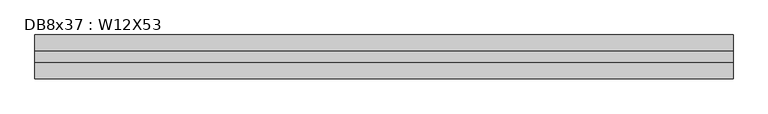
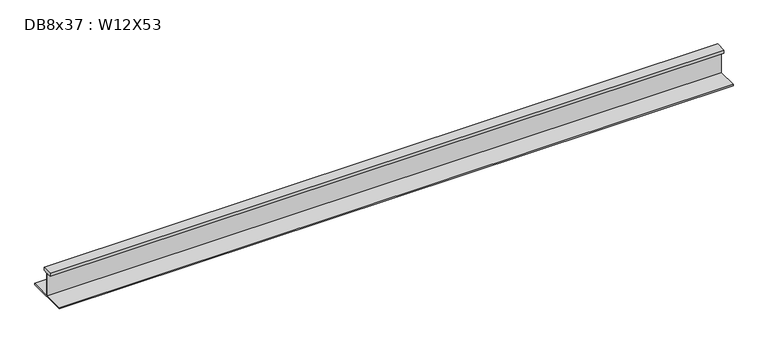
"""IFC4 building model written with IfcOpenShell, lengths in millimetres: beam geometry, DB8x37 : W12X53."""

import ifcopenshell
import ifcopenshell.guid

model = None  # the IFC model being written
_history = None  # IfcOwnerHistory: only IFC2X3 demands one
_inside = {}  # id of a spatial element -> (the spatial element, [elements in it])
_under = {}  # id of a project, library or spatial element -> (it, [spatial elements below it])
_declared = {}  # id of a project -> (the project, [libraries it declares])
_typed = {}  # id of a type object -> (the type object, [elements of that type])
_made_of = {}  # id of a material, layer set ... -> (it, [elements and type objects made of it])


def new_model(schema):
    """Start an empty IFC model of exactly this schema.

    Asked for "IFC4X3", IfcOpenShell would pick the latest addendum, in which some entities
    have other attributes; the version numbers below select the first issue.
    IFC2X3 requires an IfcOwnerHistory on every rooted entity: one is made here for all.
    """
    global model, _history
    if schema == "IFC4X3":
        model = ifcopenshell.file(schema_version=(4, 3, 0, 0))
    else:
        model = ifcopenshell.file(schema=schema)
    _inside.clear()
    _under.clear()
    _declared.clear()
    _typed.clear()
    _made_of.clear()
    _history = None
    if model.schema == "IFC2X3":
        org = make("IfcOrganization", Name="unknown")
        user = make(
            "IfcPersonAndOrganization",
            ThePerson=make("IfcPerson", FamilyName="unknown"),
            TheOrganization=org,
        )
        app = make(
            "IfcApplication",
            ApplicationDeveloper=org,
            Version="unknown",
            ApplicationFullName="unknown",
            ApplicationIdentifier="unknown",
        )
        _history = make(
            "IfcOwnerHistory",
            OwningUser=user,
            OwningApplication=app,
            ChangeAction="ADDED",
            CreationDate=0,
        )
    return model


def make(cls, **values):
    """One entity of the class cls with the attributes given. An attribute that is None is left unset."""
    return model.create_entity(
        cls, **{name: value for name, value in values.items() if value is not None}
    )


def rooted(cls, **values):
    """An entity with a GlobalId (a new one), such as an element, a storey or a relation."""
    return make(cls, GlobalId=ifcopenshell.guid.new(), OwnerHistory=_history, **values)


def si_unit(unit_type, name, prefix=None):
    """IfcSIUnit, for example si_unit("LENGTHUNIT", "METRE", prefix="MILLI")."""
    return make("IfcSIUnit", UnitType=unit_type, Prefix=prefix, Name=name)


def assignment(units):
    """IfcUnitAssignment: the units of a project."""
    return None if units is None else make("IfcUnitAssignment", Units=units)


def point(xyz):
    """IfcCartesianPoint."""
    return None if xyz is None else make("IfcCartesianPoint", Coordinates=xyz)


def direction(xyz):
    """IfcDirection."""
    return None if xyz is None else make("IfcDirection", DirectionRatios=xyz)


def frame(location, z_axis=None, x_axis=None):
    """IfcAxis2Placement3D, a coordinate frame: its origin and axes. An axis left out is left unset."""
    return make(
        "IfcAxis2Placement3D",
        Location=point(location),
        Axis=direction(z_axis),
        RefDirection=direction(x_axis),
    )


def origin():
    """The frame at (0, 0, 0) with its axes left unset."""
    return frame((0.0, 0.0, 0.0))


def place(relative_to, where):
    """IfcLocalPlacement: puts the frame where relative to a parent placement (None: the world)."""
    return make(
        "IfcLocalPlacement", PlacementRelTo=relative_to, RelativePlacement=where
    )


def context(
    kind, dimensions, precision=None, world=None, true_north=None, identifier=None
):
    """IfcGeometricRepresentationContext, for example the 3D "Model" context."""
    return make(
        "IfcGeometricRepresentationContext",
        ContextIdentifier=identifier,
        ContextType=kind,
        CoordinateSpaceDimension=dimensions,
        Precision=precision,
        WorldCoordinateSystem=world,
        TrueNorth=true_north,
    )


def project(units=None, contexts=None):
    """IfcProject with its units and contexts."""
    return rooted(
        "IfcProject",
        Name="project",
        RepresentationContexts=contexts,
        UnitsInContext=assignment(units),
    )


def spatial(cls, under=None, at=None, **own):
    """A site, building, storey or space (cls), placed at a placement, below another one or the project."""
    s = rooted(cls, ObjectPlacement=at, **own)
    if under is not None:
        _under.setdefault(under.id(), (under, []))[1].append(s)
    return s


def polyline(points):
    """IfcPolyline through the points."""
    return make("IfcPolyline", Points=[point(p) for p in points])


def outline(outer, holes=None, kind="AREA"):
    """IfcArbitraryClosedProfileDef: a profile drawn as a closed curve; with holes, ...WithVoids."""
    if holes is None:
        return make("IfcArbitraryClosedProfileDef", ProfileType=kind, OuterCurve=outer)
    return make(
        "IfcArbitraryProfileDefWithVoids",
        ProfileType=kind,
        OuterCurve=outer,
        InnerCurves=holes,
    )


def extrude(swept, where, along, depth):
    """IfcExtrudedAreaSolid: the profile swept, set in the frame where, extruded along a direction by depth."""
    return make(
        "IfcExtrudedAreaSolid",
        SweptArea=swept,
        Position=where,
        ExtrudedDirection=direction(along),
        Depth=depth,
    )


def shape(context_of_items, identifier, shape_type, items):
    """IfcShapeRepresentation: the items that make up one representation, for example the "Body"."""
    return make(
        "IfcShapeRepresentation",
        ContextOfItems=context_of_items,
        RepresentationIdentifier=identifier,
        RepresentationType=shape_type,
        Items=items,
    )


def source(mapping_origin, context_of_items, identifier, shape_type, items):
    """IfcRepresentationMap: a shape defined once, which mapped items show again and again."""
    return make(
        "IfcRepresentationMap",
        MappingOrigin=mapping_origin,
        MappedRepresentation=shape(context_of_items, identifier, shape_type, items),
    )


def transform(
    local_origin,
    x_axis=None,
    y_axis=None,
    z_axis=None,
    scale=None,
    scale2=None,
    scale3=None,
    uniform=True,
):
    """IfcCartesianTransformationOperator3D, or its non-uniform kind. x_axis, y_axis, z_axis: its Axis1, 2, 3."""
    if uniform:
        return make(
            "IfcCartesianTransformationOperator3D",
            Axis1=direction(x_axis),
            Axis2=direction(y_axis),
            LocalOrigin=point(local_origin),
            Scale=scale,
            Axis3=direction(z_axis),
        )
    return make(
        "IfcCartesianTransformationOperator3DnonUniform",
        Axis1=direction(x_axis),
        Axis2=direction(y_axis),
        LocalOrigin=point(local_origin),
        Scale=scale,
        Axis3=direction(z_axis),
        Scale2=scale2,
        Scale3=scale3,
    )


def mapped(mapping_source, mapping_target):
    """IfcMappedItem: shows the shape of a source again, moved by a transform."""
    return make(
        "IfcMappedItem", MappingSource=mapping_source, MappingTarget=mapping_target
    )


def made_of(thing, what):
    """Note that an element or type object is made of a material, layer set ...; save() writes the relation."""
    if what is not None:
        _made_of.setdefault(what.id(), (what, []))[1].append(thing)
    return thing


def element(
    cls,
    number,
    at=None,
    inside=None,
    cuts=None,
    type_object=None,
    material=None,
    context=None,
    identifier="Body",
    shape_type=None,
    held_by="IfcProductDefinitionShape",
    body=None,
    shapes=None,
    **own,
):
    """One element of the class cls, such as IfcWall. Its Tag is "e" and its number.

    at: its placement. inside: the storey or other place that contains it. cuts: it is an
    opening in that element (IfcRelVoidsElement). A single representation is given by context,
    identifier, shape_type and body (its items); several are given by shapes. held_by: the class
    of the entity that holds the representations. save() writes the other relations.
    """
    e = rooted(cls, Tag="e%d" % number, ObjectPlacement=at, **own)
    if body is not None:
        shapes = [shape(context, identifier, shape_type, body)]
    if shapes is not None:
        e.Representation = make(held_by, Representations=shapes)
    if inside is not None:
        _inside.setdefault(inside.id(), (inside, []))[1].append(e)
    if cuts is not None:
        rooted(
            "IfcRelVoidsElement", RelatingBuildingElement=cuts, RelatedOpeningElement=e
        )
    if type_object is not None:
        _typed.setdefault(type_object.id(), (type_object, []))[1].append(e)
    return made_of(e, material)


def aggregate(whole, parts):
    """IfcRelAggregates: a whole, such as a stair, and the parts it consists of."""
    return rooted("IfcRelAggregates", RelatingObject=whole, RelatedObjects=parts)


def save(model, path):
    """Write the relations noted so far, then the file.

    IfcRelAggregates (storeys below a building ...), IfcRelContainedInSpatialStructure (elements
    in a storey), IfcRelDefinesByType, IfcRelAssociatesMaterial and IfcRelDeclares: one each for
    every whole, place, type object, material and project.
    """
    for whole, parts in _under.values():
        aggregate(whole, parts)
    for where, things in _inside.values():
        rooted(
            "IfcRelContainedInSpatialStructure",
            RelatedElements=things,
            RelatingStructure=where,
        )
    for kind, things in _typed.values():
        rooted("IfcRelDefinesByType", RelatedObjects=things, RelatingType=kind)
    for what, things in _made_of.values():
        rooted("IfcRelAssociatesMaterial", RelatedObjects=things, RelatingMaterial=what)
    for by, libraries in _declared.values():
        rooted("IfcRelDeclares", RelatingContext=by, RelatedDefinitions=libraries)
    model.write(path)


def db8x37_w12x53_57ad42f3(model_context):
    return source(origin(), model_context, "Body", "SweptSolid", [
        extrude(outline(polyline([(38.1, 145.415), (38.1, 120.015), (2.921, 120.015), (2.921, -48.4505), (152.4, -48.4505), (152.4, -58.1025), (-152.4, -58.1025), (-152.4, -48.4505), (-2.921, -48.4505), (-2.921, 120.015), (-38.1, 120.015), (-38.1, 145.415), (38.1, 145.415)])), frame((-2497.8324214, 0.0, 0.0), z_axis=(1.0, 0.0, 0.0), x_axis=(0.0, 1.0, 0.0)), (0.0, 0.0, 1.0), 4871.291124),
    ])


if __name__ == "__main__":
    model = new_model("IFC4")
    model_context = context("Model", 3, world=origin())
    ifc_project = project(units=[si_unit("LENGTHUNIT", "METRE", prefix="MILLI")], contexts=[model_context])
    site = spatial("IfcSite", under=ifc_project)
    building = spatial("IfcBuilding", under=site)
    placement = place(None, origin())
    db8x37_w12x53_shape = db8x37_w12x53_57ad42f3(model_context)
    element("IfcBeam", 1, ObjectType="DB8x37 : W12X53", at=placement, inside=building, context=model_context, shape_type="MappedRepresentation", body=[
        mapped(db8x37_w12x53_shape, transform((0.0, 0.0, 0.0), x_axis=(1.0, 0.0, 0.0), y_axis=(0.0, 1.0, 0.0), z_axis=(0.0, 0.0, 1.0))),
    ])
    save(model, "model.ifc")

# Revit data of these elements
# Type "DB8x37 : W12X53"
#   Assembly Code = "B10"
#   W = 53
#   Length [instance default] = 5' - 0"
#   bf = 0' - 10"
#   d = 1' - 0.1"
#   k = 0' - 1 3/8"
#   k2 = 0' - 0.8"
#   tf = 0' - 0.575"
#   tw = 0' - 0.345"
#   A = 0.108333 SF
#   Structural Material [instance default] = Steel ASTM A992
# Element 1 (IfcBeam, "DB8x37 : W12X53")
#   Materials on its faces: "Steel ASTM A992"
# Materials
#   "Steel ASTM A992": class "Metal", colour RGB 199 199 199, transparency 0, Description = "Structural steel 50ksi", Cost = 0
